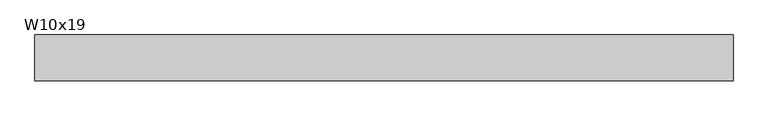
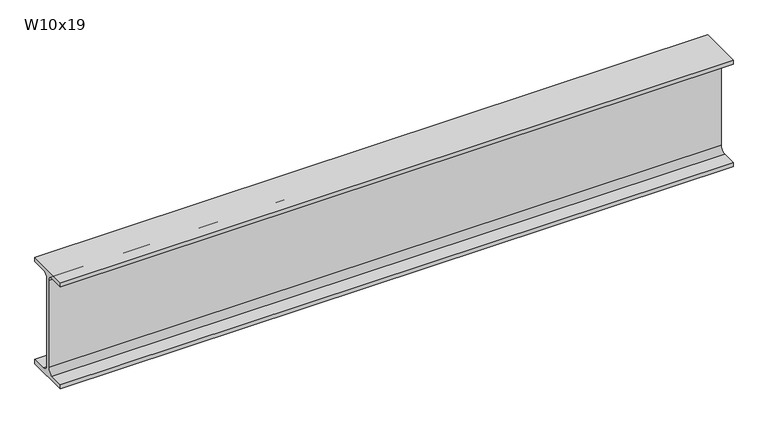
"""IFC4 building model written with IfcOpenShell, lengths in millimetres: beam geometry, RME W-Wide Flange : W10x19."""

from ifc_helpers import new_model, si_unit, point, frame, frame_2d, origin, place, context, project, spatial, polyline, circle_curve, trimmed, segment, composite_curve, outline, extrude, source, transform, mapped, element, save


def w10x19_7a1cdcd1(model_context):
    return source(origin(), model_context, "Body", "SweptSolid", [
        extrude(outline(composite_curve([segment(polyline([(51.054, -119.507), (51.054, -129.54), (-51.054, -129.54), (-51.054, -119.507), (-16.9545, -119.507)]), True, "CONTINUOUS"), segment(trimmed(circle_curve(frame_2d((-16.9545, -105.7275)), 13.7795), [point((-16.9545, -119.507))], [point((-3.175, -105.7275))], True, "CARTESIAN"), True, "CONTINUOUS"), segment(polyline([(-3.175, -105.7275), (-3.175, 105.7275)]), True, "CONTINUOUS"), segment(trimmed(circle_curve(frame_2d((-16.9545, 105.7275)), 13.7795), [point((-3.175, 105.7275))], [point((-16.9545, 119.507))], True, "CARTESIAN"), True, "CONTINUOUS"), segment(polyline([(-16.9545, 119.507), (-51.054, 119.507), (-51.054, 129.54), (51.054, 129.54), (51.054, 119.507), (16.9545, 119.507)]), True, "CONTINUOUS"), segment(trimmed(circle_curve(frame_2d((16.9545, 105.7275)), 13.7795), [point((16.9545, 119.507))], [point((3.175, 105.7275))], True, "CARTESIAN"), True, "CONTINUOUS"), segment(polyline([(3.175, 105.7275), (3.175, -105.7275)]), True, "CONTINUOUS"), segment(trimmed(circle_curve(frame_2d((16.9545, -105.7275)), 13.7795), [point((3.175, -105.7275))], [point((16.9545, -119.507))], True, "CARTESIAN"), True, "CONTINUOUS"), segment(polyline([(16.9545, -119.507), (51.054, -119.507)]), True, "CONTINUOUS")], self_intersect=False)), frame((-774.7151426, 0.0, 0.0), z_axis=(1.0, 0.0, 0.0), x_axis=(0.0, 1.0, 0.0)), (0.0, 0.0, 1.0), 1549.4302852),
    ])


if __name__ == "__main__":
    model = new_model("IFC4")
    model_context = context("Model", 3, world=origin())
    ifc_project = project(units=[si_unit("LENGTHUNIT", "METRE", prefix="MILLI")], contexts=[model_context])
    site = spatial("IfcSite", under=ifc_project)
    building = spatial("IfcBuilding", under=site)
    placement = place(None, origin())
    w10x19_shape = w10x19_7a1cdcd1(model_context)
    element("IfcBeam", 1, ObjectType="RME W-Wide Flange : W10x19", at=placement, inside=building, context=model_context, shape_type="MappedRepresentation", body=[
        mapped(w10x19_shape, transform((0.0, 0.0, 0.0), x_axis=(1.0, 0.0, 0.0), y_axis=(0.0, 1.0, 0.0), z_axis=(0.0, 0.0, 1.0))),
    ])
    save(model, "model.ifc")

# Revit data of these elements
# Type "RME W-Wide Flange : W10x19"
#   WELD P [instance default] = ""
#   WELD LE [instance default] = ""
#   WELD D [instance default] = ""
#   TOP SECTION SIZE [instance default] = ""
#   TOP SECTION LENGTH [instance default] = ""
#   REMARKS [instance default] = ""
#   REINF TYPE [instance default] = ""
#   Nominal Size = "W24"
#   End Bearing Capacity [instance default] = ""
#   BOT SECTION SIZE [instance default] = ""
#   BOT SECTION LENGTH [instance default] = ""
#   Assembly Code = "B10"
#   W = 19
#   Start Extension Calculation [instance default] = 10' - 0"
#   Start Extension [instance default] = -0' - 0 1/2"
#   End Extension Calculation [instance default] = 10' - 0"
#   End Extension [instance default] = -0' - 0 1/2"
#   Length [instance default] = 5' - 0"
#   bf = 0' - 4.02"
#   d = 0' - 10.2"
#   k = 0' - 0 15/16"
#   k2 = 0' - 0.5425"
#   tf = 0' - 0.395"
#   tw = 0' - 0 1/4"
#   A = 0.0390278 SF
#   Structural Material [instance default] = Metal - Steel - ASTM A992
# Element 1 (IfcBeam, "RME W-Wide Flange : W10x19")
#   Length = 5' - 1.00119"
#   Materials on its faces: "Metal - Steel - ASTM A992"
# Materials
#   "Metal - Steel - ASTM A992": class "Metal", colour RGB 255 128 0, transparency 0
